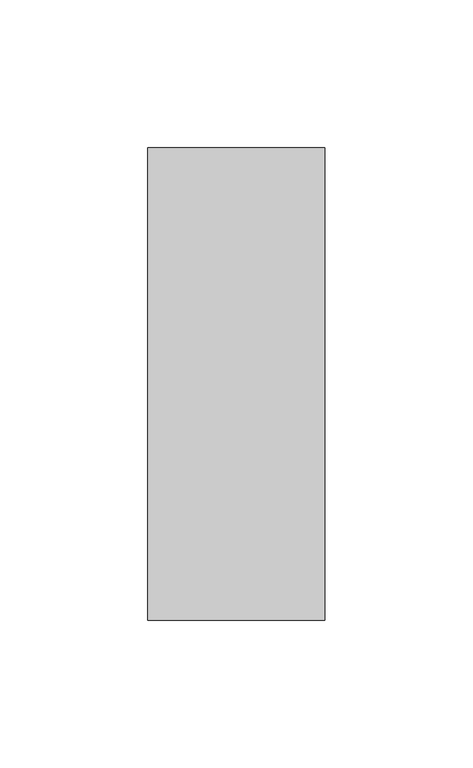
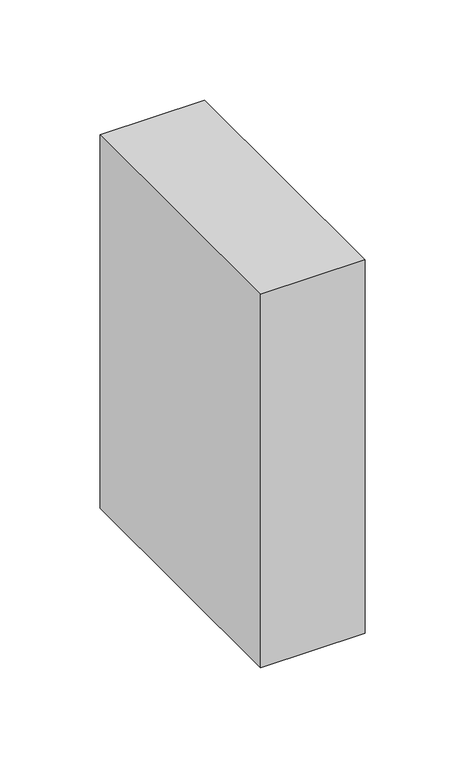
"""IFC4 building model written with IfcOpenShell, lengths in millimetres: column geometry, Madeira de lei-Coluna : Pontalete 6X16cm."""

import ifcopenshell
import ifcopenshell.guid

model = None  # the IFC model being written
_history = None  # IfcOwnerHistory: only IFC2X3 demands one
_inside = {}  # id of a spatial element -> (the spatial element, [elements in it])
_under = {}  # id of a project, library or spatial element -> (it, [spatial elements below it])
_declared = {}  # id of a project -> (the project, [libraries it declares])
_typed = {}  # id of a type object -> (the type object, [elements of that type])
_made_of = {}  # id of a material, layer set ... -> (it, [elements and type objects made of it])


def new_model(schema):
    """Start an empty IFC model of exactly this schema.

    Asked for "IFC4X3", IfcOpenShell would pick the latest addendum, in which some entities
    have other attributes; the version numbers below select the first issue.
    IFC2X3 requires an IfcOwnerHistory on every rooted entity: one is made here for all.
    """
    global model, _history
    if schema == "IFC4X3":
        model = ifcopenshell.file(schema_version=(4, 3, 0, 0))
    else:
        model = ifcopenshell.file(schema=schema)
    _inside.clear()
    _under.clear()
    _declared.clear()
    _typed.clear()
    _made_of.clear()
    _history = None
    if model.schema == "IFC2X3":
        org = make("IfcOrganization", Name="unknown")
        user = make(
            "IfcPersonAndOrganization",
            ThePerson=make("IfcPerson", FamilyName="unknown"),
            TheOrganization=org,
        )
        app = make(
            "IfcApplication",
            ApplicationDeveloper=org,
            Version="unknown",
            ApplicationFullName="unknown",
            ApplicationIdentifier="unknown",
        )
        _history = make(
            "IfcOwnerHistory",
            OwningUser=user,
            OwningApplication=app,
            ChangeAction="ADDED",
            CreationDate=0,
        )
    return model


def make(cls, **values):
    """One entity of the class cls with the attributes given. An attribute that is None is left unset."""
    return model.create_entity(
        cls, **{name: value for name, value in values.items() if value is not None}
    )


def rooted(cls, **values):
    """An entity with a GlobalId (a new one), such as an element, a storey or a relation."""
    return make(cls, GlobalId=ifcopenshell.guid.new(), OwnerHistory=_history, **values)


def si_unit(unit_type, name, prefix=None):
    """IfcSIUnit, for example si_unit("LENGTHUNIT", "METRE", prefix="MILLI")."""
    return make("IfcSIUnit", UnitType=unit_type, Prefix=prefix, Name=name)


def assignment(units):
    """IfcUnitAssignment: the units of a project."""
    return None if units is None else make("IfcUnitAssignment", Units=units)


def point(xyz):
    """IfcCartesianPoint."""
    return None if xyz is None else make("IfcCartesianPoint", Coordinates=xyz)


def direction(xyz):
    """IfcDirection."""
    return None if xyz is None else make("IfcDirection", DirectionRatios=xyz)


def frame(location, z_axis=None, x_axis=None):
    """IfcAxis2Placement3D, a coordinate frame: its origin and axes. An axis left out is left unset."""
    return make(
        "IfcAxis2Placement3D",
        Location=point(location),
        Axis=direction(z_axis),
        RefDirection=direction(x_axis),
    )


def origin():
    """The frame at (0, 0, 0) with its axes left unset."""
    return frame((0.0, 0.0, 0.0))


def place(relative_to, where):
    """IfcLocalPlacement: puts the frame where relative to a parent placement (None: the world)."""
    return make(
        "IfcLocalPlacement", PlacementRelTo=relative_to, RelativePlacement=where
    )


def context(
    kind, dimensions, precision=None, world=None, true_north=None, identifier=None
):
    """IfcGeometricRepresentationContext, for example the 3D "Model" context."""
    return make(
        "IfcGeometricRepresentationContext",
        ContextIdentifier=identifier,
        ContextType=kind,
        CoordinateSpaceDimension=dimensions,
        Precision=precision,
        WorldCoordinateSystem=world,
        TrueNorth=true_north,
    )


def project(units=None, contexts=None):
    """IfcProject with its units and contexts."""
    return rooted(
        "IfcProject",
        Name="project",
        RepresentationContexts=contexts,
        UnitsInContext=assignment(units),
    )


def spatial(cls, under=None, at=None, **own):
    """A site, building, storey or space (cls), placed at a placement, below another one or the project."""
    s = rooted(cls, ObjectPlacement=at, **own)
    if under is not None:
        _under.setdefault(under.id(), (under, []))[1].append(s)
    return s


def polyline(points):
    """IfcPolyline through the points."""
    return make("IfcPolyline", Points=[point(p) for p in points])


def outline(outer, holes=None, kind="AREA"):
    """IfcArbitraryClosedProfileDef: a profile drawn as a closed curve; with holes, ...WithVoids."""
    if holes is None:
        return make("IfcArbitraryClosedProfileDef", ProfileType=kind, OuterCurve=outer)
    return make(
        "IfcArbitraryProfileDefWithVoids",
        ProfileType=kind,
        OuterCurve=outer,
        InnerCurves=holes,
    )


def extrude(swept, where, along, depth):
    """IfcExtrudedAreaSolid: the profile swept, set in the frame where, extruded along a direction by depth."""
    return make(
        "IfcExtrudedAreaSolid",
        SweptArea=swept,
        Position=where,
        ExtrudedDirection=direction(along),
        Depth=depth,
    )


def shape(context_of_items, identifier, shape_type, items):
    """IfcShapeRepresentation: the items that make up one representation, for example the "Body"."""
    return make(
        "IfcShapeRepresentation",
        ContextOfItems=context_of_items,
        RepresentationIdentifier=identifier,
        RepresentationType=shape_type,
        Items=items,
    )


def source(mapping_origin, context_of_items, identifier, shape_type, items):
    """IfcRepresentationMap: a shape defined once, which mapped items show again and again."""
    return make(
        "IfcRepresentationMap",
        MappingOrigin=mapping_origin,
        MappedRepresentation=shape(context_of_items, identifier, shape_type, items),
    )


def transform(
    local_origin,
    x_axis=None,
    y_axis=None,
    z_axis=None,
    scale=None,
    scale2=None,
    scale3=None,
    uniform=True,
):
    """IfcCartesianTransformationOperator3D, or its non-uniform kind. x_axis, y_axis, z_axis: its Axis1, 2, 3."""
    if uniform:
        return make(
            "IfcCartesianTransformationOperator3D",
            Axis1=direction(x_axis),
            Axis2=direction(y_axis),
            LocalOrigin=point(local_origin),
            Scale=scale,
            Axis3=direction(z_axis),
        )
    return make(
        "IfcCartesianTransformationOperator3DnonUniform",
        Axis1=direction(x_axis),
        Axis2=direction(y_axis),
        LocalOrigin=point(local_origin),
        Scale=scale,
        Axis3=direction(z_axis),
        Scale2=scale2,
        Scale3=scale3,
    )


def mapped(mapping_source, mapping_target):
    """IfcMappedItem: shows the shape of a source again, moved by a transform."""
    return make(
        "IfcMappedItem", MappingSource=mapping_source, MappingTarget=mapping_target
    )


def made_of(thing, what):
    """Note that an element or type object is made of a material, layer set ...; save() writes the relation."""
    if what is not None:
        _made_of.setdefault(what.id(), (what, []))[1].append(thing)
    return thing


def element(
    cls,
    number,
    at=None,
    inside=None,
    cuts=None,
    type_object=None,
    material=None,
    context=None,
    identifier="Body",
    shape_type=None,
    held_by="IfcProductDefinitionShape",
    body=None,
    shapes=None,
    **own,
):
    """One element of the class cls, such as IfcWall. Its Tag is "e" and its number.

    at: its placement. inside: the storey or other place that contains it. cuts: it is an
    opening in that element (IfcRelVoidsElement). A single representation is given by context,
    identifier, shape_type and body (its items); several are given by shapes. held_by: the class
    of the entity that holds the representations. save() writes the other relations.
    """
    e = rooted(cls, Tag="e%d" % number, ObjectPlacement=at, **own)
    if body is not None:
        shapes = [shape(context, identifier, shape_type, body)]
    if shapes is not None:
        e.Representation = make(held_by, Representations=shapes)
    if inside is not None:
        _inside.setdefault(inside.id(), (inside, []))[1].append(e)
    if cuts is not None:
        rooted(
            "IfcRelVoidsElement", RelatingBuildingElement=cuts, RelatedOpeningElement=e
        )
    if type_object is not None:
        _typed.setdefault(type_object.id(), (type_object, []))[1].append(e)
    return made_of(e, material)


def aggregate(whole, parts):
    """IfcRelAggregates: a whole, such as a stair, and the parts it consists of."""
    return rooted("IfcRelAggregates", RelatingObject=whole, RelatedObjects=parts)


def save(model, path):
    """Write the relations noted so far, then the file.

    IfcRelAggregates (storeys below a building ...), IfcRelContainedInSpatialStructure (elements
    in a storey), IfcRelDefinesByType, IfcRelAssociatesMaterial and IfcRelDeclares: one each for
    every whole, place, type object, material and project.
    """
    for whole, parts in _under.values():
        aggregate(whole, parts)
    for where, things in _inside.values():
        rooted(
            "IfcRelContainedInSpatialStructure",
            RelatedElements=things,
            RelatingStructure=where,
        )
    for kind, things in _typed.values():
        rooted("IfcRelDefinesByType", RelatedObjects=things, RelatingType=kind)
    for what, things in _made_of.values():
        rooted("IfcRelAssociatesMaterial", RelatedObjects=things, RelatingMaterial=what)
    for by, libraries in _declared.values():
        rooted("IfcRelDeclares", RelatingContext=by, RelatedDefinitions=libraries)
    model.write(path)


def column_42eef9f8(model_context):
    return source(origin(), model_context, "Body", "SweptSolid", [
        extrude(outline(polyline([(30.0, 80.0), (30.0, -80.0), (-30.0, -80.0), (-30.0, 80.0), (30.0, 80.0)])), frame((0.0, 0.0, 6710.0), z_axis=(0.0, 0.0, 1.0), x_axis=(1.0, 0.0, 0.0)), (0.0, 0.0, 1.0), 227.1),
    ])


if __name__ == "__main__":
    model = new_model("IFC4")
    model_context = context("Model", 3, world=origin())
    ifc_project = project(units=[si_unit("LENGTHUNIT", "METRE", prefix="MILLI")], contexts=[model_context])
    site = spatial("IfcSite", under=ifc_project)
    building = spatial("IfcBuilding", under=site)
    placement = place(None, origin())
    column_shape = column_42eef9f8(model_context)
    element("IfcColumn", 1, ObjectType="Madeira de lei-Coluna : Pontalete 6X16cm", at=placement, inside=building, context=model_context, shape_type="MappedRepresentation", body=[
        mapped(column_shape, transform((0.0, 0.0, 0.0), x_axis=(1.0, 0.0, 0.0), y_axis=(0.0, 1.0, 0.0), z_axis=(0.0, 0.0, 1.0))),
    ])
    save(model, "model.ifc")

# Revit data of these elements
# Type "Madeira de lei-Coluna : Pontalete 6X16cm"
#   A = 0.01952 m²
#   b = 0.06 m
#   d = 0.16 m
#   Structural Material [instance default] = none
#   Assembly Code = ""
# Element 1 (IfcColumn, "Madeira de lei-Coluna : Pontalete 6X16cm")
#   Structural Material = .MADEIRAMENTO
#   Materials on its faces: ".MADEIRAMENTO"
# Materials
#   ".MADEIRAMENTO": class ".CC_MADEIRAS", colour RGB 212 179 113, transparency 0, Cost = 0
